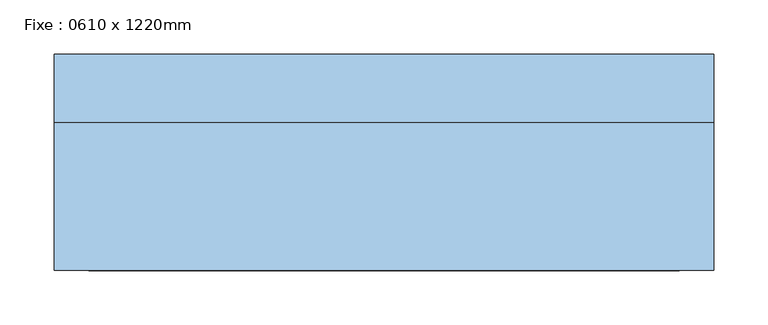
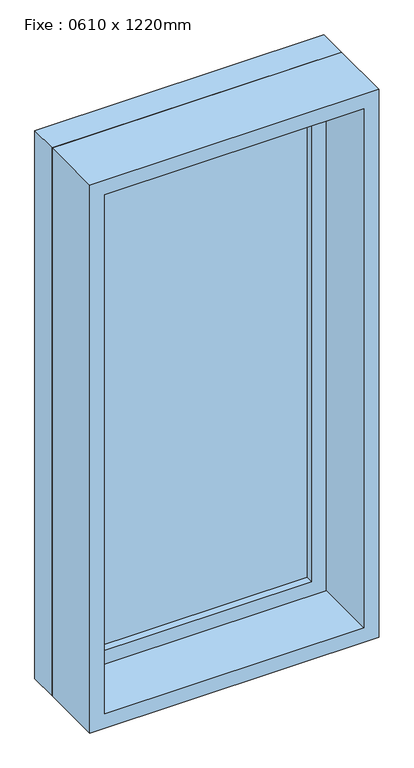
"""IFC4 building model written with IfcOpenShell, lengths in millimetres: window geometry, Fixe : 0610 x 1220mm."""

from ifc_helpers import new_model, si_unit, frame, origin, place, context, project, spatial, polyline, outline, extrude, source, transform, mapped, element, save


def fixe_0610_x_1220mm_4e981104(model_context):
    return source(origin(), model_context, "Body", "SweptSolid", [
        extrude(outline(polyline([(-242.0, 78.0), (242.0, 78.0), (242.0, 66.0), (-242.0, 66.0), (-242.0, 78.0)])), frame((0.0, 0.0, 978.0), z_axis=(0.0, 0.0, 1.0), x_axis=(1.0, 0.0, 0.0)), (0.0, 0.0, 1.0), 1094.0),
        extrude(outline(polyline([(2116.0, -286.0), (934.0, -286.0), (934.0, 286.0), (2116.0, 286.0), (2116.0, -286.0)]), holes=[polyline([(2072.0, -242.0), (2072.0, 242.0), (978.0, 242.0), (978.0, -242.0), (2072.0, -242.0)])]), frame((0.0, 50.0, 0.0), z_axis=(0.0, 1.0, 0.0), x_axis=(0.0, 0.0, 1.0)), (0.0, 0.0, 1.0), 44.0),
        extrude(outline(polyline([(2135.0, -305.0), (915.0, -305.0), (915.0, 305.0), (2135.0, 305.0), (2135.0, -305.0)]), holes=[polyline([(2116.0, -286.0), (2116.0, 286.0), (934.0, 286.0), (934.0, -286.0), (2116.0, -286.0)])]), frame((0.0, 50.0, 0.0), z_axis=(0.0, 1.0, 0.0), x_axis=(0.0, 0.0, 1.0)), (0.0, 0.0, 1.0), 63.0),
        extrude(outline(polyline([(2135.0, -305.0), (915.0, -305.0), (915.0, 305.0), (2135.0, 305.0), (2135.0, -305.0)]), holes=[polyline([(2103.0, -273.0), (2103.0, 273.0), (947.0, 273.0), (947.0, -273.0), (2103.0, -273.0)])]), frame((0.0, -87.0, 0.0), z_axis=(0.0, 1.0, 0.0), x_axis=(0.0, 0.0, 1.0)), (0.0, 0.0, 1.0), 137.0),
    ])


if __name__ == "__main__":
    model = new_model("IFC4")
    model_context = context("Model", 3, world=origin())
    ifc_project = project(units=[si_unit("LENGTHUNIT", "METRE", prefix="MILLI")], contexts=[model_context])
    site = spatial("IfcSite", under=ifc_project)
    building = spatial("IfcBuilding", under=site)
    placement = place(None, origin())
    fixe_0610_x_1220mm_shape = fixe_0610_x_1220mm_4e981104(model_context)
    element("IfcWindow", 1, ObjectType="Fixe : 0610 x 1220mm", at=placement, inside=building, context=model_context, shape_type="MappedRepresentation", body=[
        mapped(fixe_0610_x_1220mm_shape, transform((0.0, 0.0, 0.0), x_axis=(1.0, 0.0, 0.0), y_axis=(0.0, 1.0, 0.0), z_axis=(0.0, 0.0, 1.0))),
    ])
    save(model, "model.ifc")

# Revit data of these elements
# Type "Fixe : 0610 x 1220mm"
#   Type Mark = "13"
#   Construction Type Id = "GSP4R"
#   Analytic Construction = "Simple vitrage Pilkington 1/8 po."
#   Visual Light Transmittance = 0.9
#   Solar Heat Gain Coefficient = 0.78
#   Heat Transfer Coefficient (U) = 3.6886 W/(m²·K)
#   Height = 1.22 m
#   Hauteur de l'appui par défaut = 0.915 m
#   Width = 0.61 m
#   Encastrement de fenêtre = 0.019 m
#   Define Thermal Properties by = 1
#   Matériau de cadre extérieur = Châssis
#   Matériau du cadre intérieur = Châssis
#   Matériau du panneau de verre = Verre
#   Châssis = Châssis
#   Wall Closure = (empty or 0)
# Element 1 (IfcWindow, "Fixe : 0610 x 1220mm")
#   Materials on its faces: "Châssis", "Verre"
# Materials
#   "Châssis": class "Bois", colour RGB 224 178 126, transparency 0, Cost = 0
#   "Verre": class "Verre", colour RGB 0 128 192, transparency 0.9, Description = "Verre sodocalcique", Cost = 0
